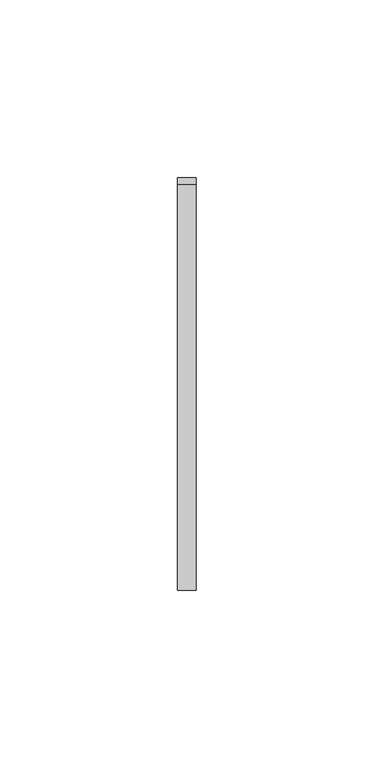
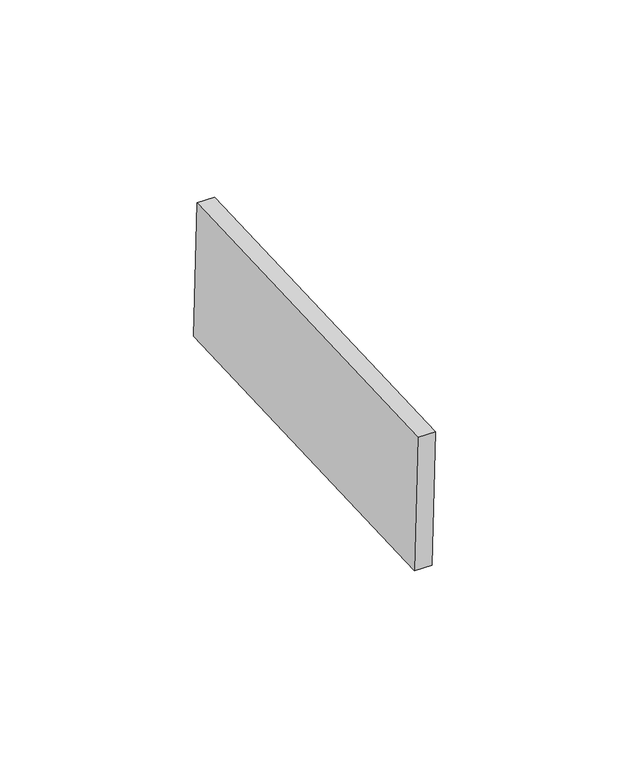
"""IFC4 building model written with IfcOpenShell, lengths in millimetres: proxy geometry, Inner panel:Inner panel:1:Inner panel:1 : Inner panel:Inner panel:300324:2:Inner panel:1:Inner panel:1 : Inner panel:Inner panel:300324:2 : Inner panel:Inner panel:1:Inner panel:1 : Inner panel:Inner panel:300324:300043:91 : Inner panel:Inner panel:1:Inner panel:1 : Inner panel:Inner panel:300324:2:Inner panel:1:Inner panel:1 : Inner panel:Inner panel:300324:2 : Inner panel:Inner panel:1:Inner panel:1 : Inner panel:Inner panel:300324:300043:308120."""

from ifc_helpers import new_model, si_unit, frame, origin, place, context, project, spatial, polyline, outline, extrude, source, transform, mapped, element, save


def generic_models_4818c94b(model_context):
    return source(origin(), model_context, "Body", "SweptSolid", [
        extrude(outline(polyline([(0.0, -114.2999999), (0.0, 0.0), (5.2138089, 0.0), (5.2138089, -114.2999999), (0.0, -114.2999999)])), frame((591904.595117, -568168.273882, 8806.9397902), z_axis=(0.0, -0.04163054471215927, 0.9991330730923529), x_axis=(-1.0, 0.0, 0.0)), (0.0, 0.0, 1.0), 43.2233908),
    ])


if __name__ == "__main__":
    model = new_model("IFC4")
    model_context = context("Model", 3, world=origin())
    ifc_project = project(units=[si_unit("LENGTHUNIT", "METRE", prefix="MILLI")], contexts=[model_context])
    site = spatial("IfcSite", under=ifc_project)
    building = spatial("IfcBuilding", under=site)
    placement = place(None, origin())
    generic_models_shape = generic_models_4818c94b(model_context)
    element("IfcBuildingElementProxy", 1, Name="Inner panel:Inner panel:1:Inner panel:1 : Inner panel:Inner panel:300324:2:Inner panel:1:Inner panel:1 : Inner panel:Inner panel:300324:2 : Inner panel:Inner panel:1:Inner panel:1 : Inner panel:Inner panel:300324:300043:91 : Inner panel:Inner panel:1:Inner panel:1 : Inner panel:Inner panel:300324:2:Inner panel:1:Inner panel:1 : Inner panel:Inner panel:300324:2 : Inner panel:Inner panel:1:Inner panel:1 : Inner panel:Inner panel:300324:300043:308120", ObjectType="Inner panel:Inner panel:1:Inner panel:1 : Inner panel:Inner panel:300324:2:Inner panel:1:Inner panel:1 : Inner panel:Inner panel:300324:2 : Inner panel:Inner panel:1:Inner panel:1 : Inner panel:Inner panel:300324:300043:91 : Inner panel:Inner panel:1:Inner panel:1 : Inner panel:Inner panel:300324:2:Inner panel:1:Inner panel:1 : Inner panel:Inner panel:300324:2 : Inner panel:Inner panel:1:Inner panel:1 : Inner panel:Inner panel:300324:300043:308120", at=placement, inside=building, context=model_context, shape_type="MappedRepresentation", body=[
        mapped(generic_models_shape, transform((0.0, 0.0, 0.0), x_axis=(1.0, 0.0, 0.0), y_axis=(0.0, 1.0, 0.0), z_axis=(0.0, 0.0, 1.0))),
    ])
    save(model, "model.ifc")

# Revit data of these elements
# Type "Inner panel:Inner panel:1:Inner panel:1 : Inner panel:Inner panel:300324:2:Inner panel:1:Inner panel:1 : Inner panel:Inner panel:300324:2 : Inner panel:Inner panel:1:Inner panel:1 : Inner panel:Inner panel:300324:300043:91 : Inner panel:Inner panel:1:Inner panel:1 : Inner panel:Inner panel:300324:2:Inner panel:1:Inner panel:1 : Inner panel:Inner panel:300324:2 : Inner panel:Inner panel:1:Inner panel:1 : Inner panel:Inner panel:300324:300043:308120"
#   NameOverride = "Inner panel:Inner panel:1:Inner panel:1 : Inner panel:Inner panel:300324:2:Inner panel:1:Inner panel:1 : Inner panel:Inner panel:300324:2 : Inner panel:Inner panel:1:Inner panel:1 : Inner panel:Inner panel:300324:300043:308120"
#   ObjectTypeOverride = "Inner panel:1:Inner panel:1 : Inner panel:Inner panel:300324:2 : Inner panel:Inner panel:1:Inner panel:1 : Inner panel:Inner panel:300324:300043"
#   Reference = "Inner panel"
#   Tag = "308120"
# Element 1 (IfcBuildingElementProxy, "Inner panel:Inner panel:1:Inner panel:1 : Inner panel:Inner panel:300324:2:Inner panel:1:Inner panel:1 : Inner panel:Inner panel:300324:2 : Inner panel:Inner panel:1:Inner panel:1 : Inner panel:Inner panel:300324:300043:91 : Inner panel:Inner panel:1:Inner panel:1 : Inner panel:Inner panel:300324:2:Inner panel:1:Inner panel:1 : Inner panel:Inner panel:300324:2 : Inner panel:Inner panel:1:Inner panel:1 : Inner panel:Inner panel:300324:300043:308120")
#   Materials on its faces: "SLIDING CLIP"
# Materials
#   "SLIDING CLIP": class "Generic", colour RGB 120 120 120, transparency 0, Cost = 0
